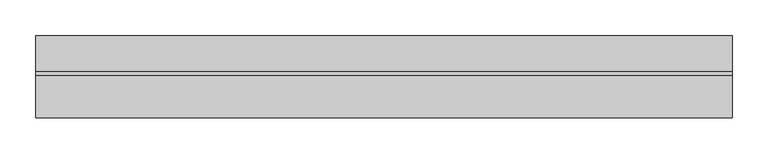
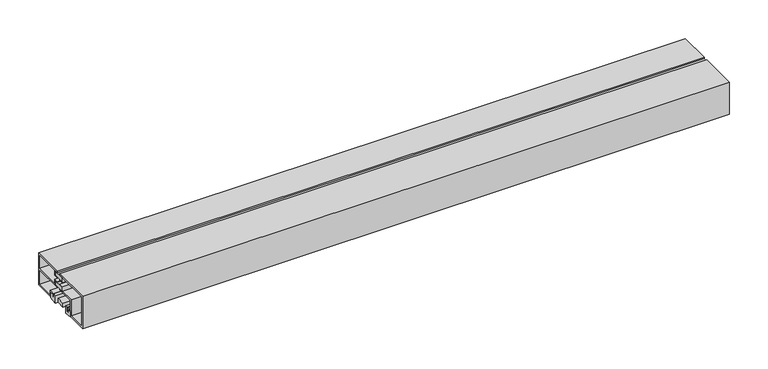
"""IFC4 building model written with IfcOpenShell, lengths in millimetres: proxy geometry, Generic Models 3:Generic Models 1:4:Generic Models 1:4 : Generic Models 3:Generic Models 1:300625:338780:Generic Models 1:4:Generic Models 1:4 : Generic Models 3:Generic Models 1:300625:338780 : Generic Models 3:Generic Models 1:4:Generic Models 1:4 : Generic Models 3:Generic Models 1:300625:338780:1 : Generic Models 3:Generic Models 1:4:Generic Models 1:4 : Generic Models 3:Generic Models 1:300625:338780:Generic Models 1:4:Generic Models 1:4 : Generic Models 3:Generic Models 1:300625:338780 : Generic Models 3:Generic Models 1:4:Generic Models 1:4 : Generic Models 3:Generic Models 1:300625:338780:301383."""

from ifc_helpers import new_model, si_unit, frame, origin, place, context, project, spatial, polyline, outline, extrude, source, transform, mapped, element, save


def generic_models_7e7e62c1(model_context):
    return source(origin(), model_context, "Body", "SweptSolid", [
        extrude(outline(polyline([(593731.7367239, -579047.9760005), (593731.7367239, -579064.0874367), (592761.7742239, -579064.0874367), (592761.7742239, -579047.9760005), (593731.7367239, -579047.9760005)])), frame((0.0, 0.0, 3693.6142952), z_axis=(0.0, 0.0, 1.0), x_axis=(1.0, 0.0, 0.0)), (0.0, 0.0, 1.0), 6.0797872),
        extrude(outline(polyline([(593731.7367239, -579047.8857325), (593731.7367239, -579063.9971687), (592761.7742239, -579063.9971687), (592761.7742239, -579047.8857325), (593731.7367239, -579047.8857325)])), frame((0.0, 0.0, 3678.5668218), z_axis=(0.0, 0.0, 1.0), x_axis=(1.0, 0.0, 0.0)), (0.0, 0.0, 1.0), 6.0797872),
        extrude(outline(polyline([(593731.7367239, -579054.6832724), (593731.7367239, -579067.3832724), (592761.7742239, -579067.3832724), (592761.7742239, -579054.6832724), (593731.7367239, -579054.6832724)])), frame((0.0, 0.0, 3654.1359064), z_axis=(0.0, 0.0, 1.0), x_axis=(1.0, 0.0, 0.0)), (0.0, 0.0, 1.0), 6.3435484),
        extrude(outline(polyline([(-579086.0195091, 3650.2669395), (-579086.0195091, 3658.1066489), (-579081.7214373, 3658.1066489), (-579081.7214373, 3655.1627892), (-579078.8757591, 3655.1627892), (-579078.8757591, 3660.8763298), (-579074.1217032, 3660.8763298), (-579074.1217032, 3648.8060727), (-579086.0195091, 3650.2669395)])), frame((592761.7742239, 0.0, 0.0), z_axis=(1.0, 0.0, 0.0), x_axis=(0.0, 1.0, 0.0)), (0.0, 0.0, 1.0), 969.9625),
        extrude(outline(polyline([(-579043.1907857, 3655.1627892), (-579040.3451075, 3655.1627892), (-579040.3451075, 3658.1066489), (-579036.0470357, 3658.1066489), (-579036.0470357, 3650.2669395), (-579047.9448415, 3648.8060727), (-579047.9448415, 3660.8763298), (-579043.1907857, 3660.8763298), (-579043.1907857, 3655.1627892)])), frame((592761.7742239, 0.0, 0.0), z_axis=(1.0, 0.0, 0.0), x_axis=(0.0, 1.0, 0.0)), (0.0, 0.0, 1.0), 969.9625),
        extrude(outline(polyline([(-579003.8663841, 3651.2837766), (-579035.6501607, 3651.2837766), (-579035.6501607, 3658.5035239), (-579040.7419825, 3658.5035239), (-579040.7419825, 3655.5596642), (-579042.7939107, 3655.5596642), (-579042.7939107, 3660.4794548), (-579033.7502272, 3660.4794548), (-579033.7502272, 3653.1935757), (-579005.8423149, 3653.1935757), (-579005.8423149, 3676.6668883), (-579052.7495623, 3676.6668883), (-579052.7495623, 3678.5668218), (-579047.8857325, 3678.5668218), (-579047.8857325, 3684.646609), (-579052.7495623, 3684.646609), (-579052.7495623, 3685.9385638), (-579045.985799, 3685.9385638), (-579045.985799, 3678.5668218), (-579005.8423149, 3678.5668218), (-579005.8423149, 3700.1277874), (-579046.076067, 3700.1277874), (-579046.076067, 3692.3223404), (-579052.8398303, 3692.3223404), (-579052.8398303, 3693.6142952), (-579047.9760005, 3693.6142952), (-579047.9760005, 3699.6940824), (-579052.8398303, 3699.6940824), (-579052.8398303, 3702.05), (-579003.8663841, 3702.05), (-579003.8663841, 3651.2837766)])), frame((592761.7742239, 0.0, 0.0), z_axis=(1.0, 0.0, 0.0), x_axis=(0.0, 1.0, 0.0)), (0.0, 0.0, 1.0), 969.9625),
        extrude(outline(polyline([(-579081.3245623, 3658.5035239), (-579086.4163841, 3658.5035239), (-579086.4163841, 3651.2837766), (-579118.1663841, 3651.2837766), (-579118.1663841, 3702.05), (-579059.2236069, 3702.05), (-579059.2236069, 3699.6940824), (-579064.0874367, 3699.6940824), (-579064.0874367, 3693.6142952), (-579059.2236069, 3693.6142952), (-579059.2236069, 3692.3223404), (-579065.9873702, 3692.3223404), (-579065.9873702, 3700.1500665), (-579115.6584719, 3700.1500665), (-579115.6584719, 3653.1837101), (-579088.3163176, 3653.1837101), (-579088.3163176, 3678.5668218), (-579065.8971022, 3678.5668218), (-579065.8971022, 3685.9385638), (-579059.1333389, 3685.9385638), (-579059.1333389, 3684.646609), (-579063.9971687, 3684.646609), (-579063.9971687, 3678.5668218), (-579059.1333389, 3678.5668218), (-579059.1333389, 3676.6668883), (-579086.4163841, 3676.6668883), (-579086.4163841, 3660.4794548), (-579079.2726341, 3660.4794548), (-579079.2726341, 3655.5596642), (-579081.3245623, 3655.5596642), (-579081.3245623, 3658.5035239)])), frame((592761.7742239, 0.0, 0.0), z_axis=(1.0, 0.0, 0.0), x_axis=(0.0, 1.0, 0.0)), (0.0, 0.0, 1.0), 969.9625),
    ])


if __name__ == "__main__":
    model = new_model("IFC4")
    model_context = context("Model", 3, world=origin())
    ifc_project = project(units=[si_unit("LENGTHUNIT", "METRE", prefix="MILLI")], contexts=[model_context])
    site = spatial("IfcSite", under=ifc_project)
    building = spatial("IfcBuilding", under=site)
    placement = place(None, origin())
    generic_models_shape = generic_models_7e7e62c1(model_context)
    element("IfcBuildingElementProxy", 1, Name="Generic Models 3:Generic Models 1:4:Generic Models 1:4 : Generic Models 3:Generic Models 1:300625:338780:Generic Models 1:4:Generic Models 1:4 : Generic Models 3:Generic Models 1:300625:338780 : Generic Models 3:Generic Models 1:4:Generic Models 1:4 : Generic Models 3:Generic Models 1:300625:338780:1 : Generic Models 3:Generic Models 1:4:Generic Models 1:4 : Generic Models 3:Generic Models 1:300625:338780:Generic Models 1:4:Generic Models 1:4 : Generic Models 3:Generic Models 1:300625:338780 : Generic Models 3:Generic Models 1:4:Generic Models 1:4 : Generic Models 3:Generic Models 1:300625:338780:301383", ObjectType="Generic Models 3:Generic Models 1:4:Generic Models 1:4 : Generic Models 3:Generic Models 1:300625:338780:Generic Models 1:4:Generic Models 1:4 : Generic Models 3:Generic Models 1:300625:338780 : Generic Models 3:Generic Models 1:4:Generic Models 1:4 : Generic Models 3:Generic Models 1:300625:338780:1 : Generic Models 3:Generic Models 1:4:Generic Models 1:4 : Generic Models 3:Generic Models 1:300625:338780:Generic Models 1:4:Generic Models 1:4 : Generic Models 3:Generic Models 1:300625:338780 : Generic Models 3:Generic Models 1:4:Generic Models 1:4 : Generic Models 3:Generic Models 1:300625:338780:301383", at=placement, inside=building, context=model_context, shape_type="MappedRepresentation", body=[
        mapped(generic_models_shape, transform((0.0, 0.0, 0.0), x_axis=(1.0, 0.0, 0.0), y_axis=(0.0, 1.0, 0.0), z_axis=(0.0, 0.0, 1.0))),
    ])
    save(model, "model.ifc")

# Revit data of these elements
# Type "Generic Models 3:Generic Models 1:4:Generic Models 1:4 : Generic Models 3:Generic Models 1:300625:338780:Generic Models 1:4:Generic Models 1:4 : Generic Models 3:Generic Models 1:300625:338780 : Generic Models 3:Generic Models 1:4:Generic Models 1:4 : Generic Models 3:Generic Models 1:300625:338780:1 : Generic Models 3:Generic Models 1:4:Generic Models 1:4 : Generic Models 3:Generic Models 1:300625:338780:Generic Models 1:4:Generic Models 1:4 : Generic Models 3:Generic Models 1:300625:338780 : Generic Models 3:Generic Models 1:4:Generic Models 1:4 : Generic Models 3:Generic Models 1:300625:338780:301383"
#   NameOverride = "Generic Models 3:Generic Models 1:4:Generic Models 1:4 : Generic Models 3:Generic Models 1:300625:338780:Generic Models 1:4:Generic Models 1:4 : Generic Models 3:Generic Models 1:300625:338780 : Generic Models 3:Generic Models 1:4:Generic Models 1:4 : Generic Models 3:Generic Models 1:300625:338780:301383"
#   ObjectTypeOverride = "Generic Models 1:4:Generic Models 1:4 : Generic Models 3:Generic Models 1:300625:338780 : Generic Models 3:Generic Models 1:4:Generic Models 1:4 : Generic Models 3:Generic Models 1:300625:338780"
#   Reference = "Generic Models 1"
#   Tag = "301383"
# Element 1 (IfcBuildingElementProxy, "Generic Models 3:Generic Models 1:4:Generic Models 1:4 : Generic Models 3:Generic Models 1:300625:338780:Generic Models 1:4:Generic Models 1:4 : Generic Models 3:Generic Models 1:300625:338780 : Generic Models 3:Generic Models 1:4:Generic Models 1:4 : Generic Models 3:Generic Models 1:300625:338780:1 : Generic Models 3:Generic Models 1:4:Generic Models 1:4 : Generic Models 3:Generic Models 1:300625:338780:Generic Models 1:4:Generic Models 1:4 : Generic Models 3:Generic Models 1:300625:338780 : Generic Models 3:Generic Models 1:4:Generic Models 1:4 : Generic Models 3:Generic Models 1:300625:338780:301383")
#   Materials on its faces: "THERMAL BROKEN ALUMINUM STOREFRONT"
# Materials
#   "THERMAL BROKEN ALUMINUM STOREFRONT": class "Unassigned", colour RGB 244 244 244, transparency 0, Cost = 0
